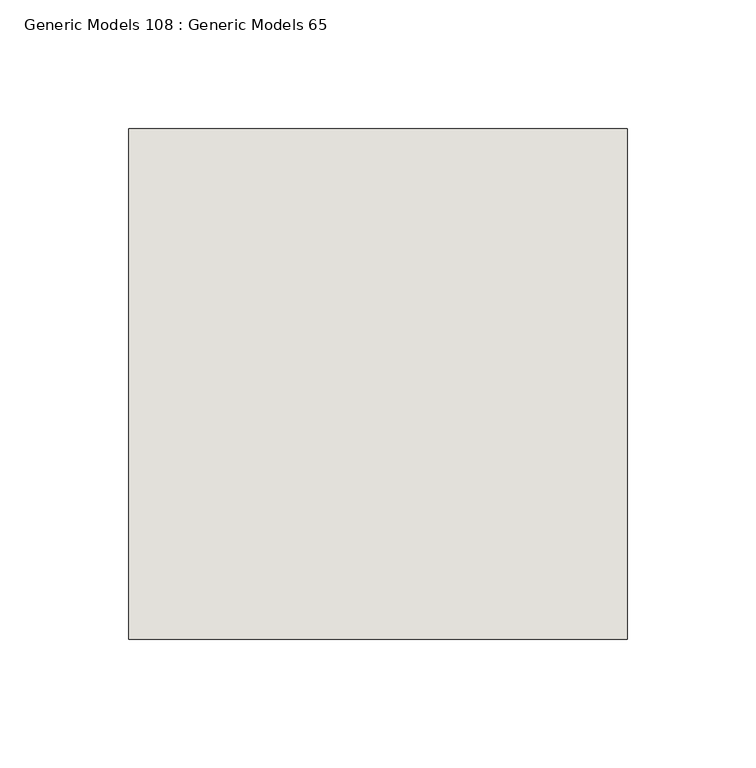
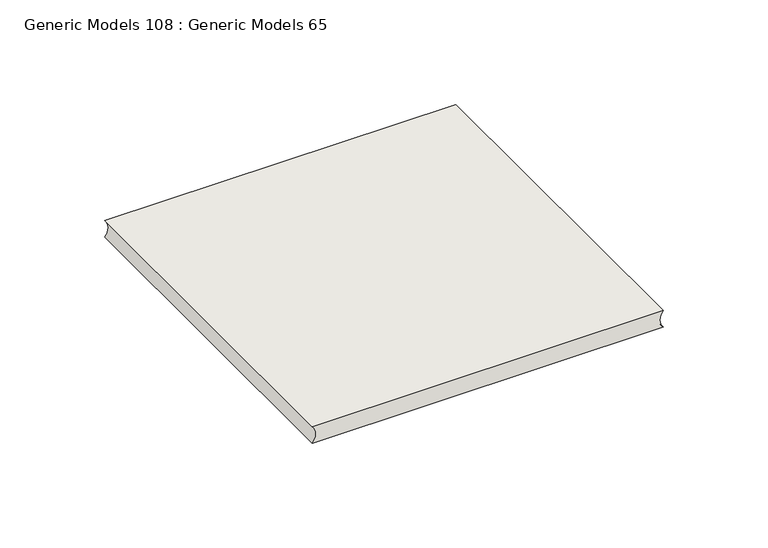
"""IFC4 building model written with IfcOpenShell, lengths in millimetres: wall geometry, Generic Models 108 : Generic Models 65."""

import ifcopenshell
import ifcopenshell.guid

model = None  # the IFC model being written
_history = None  # IfcOwnerHistory: only IFC2X3 demands one
_inside = {}  # id of a spatial element -> (the spatial element, [elements in it])
_under = {}  # id of a project, library or spatial element -> (it, [spatial elements below it])
_declared = {}  # id of a project -> (the project, [libraries it declares])
_typed = {}  # id of a type object -> (the type object, [elements of that type])
_made_of = {}  # id of a material, layer set ... -> (it, [elements and type objects made of it])


def new_model(schema):
    """Start an empty IFC model of exactly this schema.

    Asked for "IFC4X3", IfcOpenShell would pick the latest addendum, in which some entities
    have other attributes; the version numbers below select the first issue.
    IFC2X3 requires an IfcOwnerHistory on every rooted entity: one is made here for all.
    """
    global model, _history
    if schema == "IFC4X3":
        model = ifcopenshell.file(schema_version=(4, 3, 0, 0))
    else:
        model = ifcopenshell.file(schema=schema)
    _inside.clear()
    _under.clear()
    _declared.clear()
    _typed.clear()
    _made_of.clear()
    _history = None
    if model.schema == "IFC2X3":
        org = make("IfcOrganization", Name="unknown")
        user = make(
            "IfcPersonAndOrganization",
            ThePerson=make("IfcPerson", FamilyName="unknown"),
            TheOrganization=org,
        )
        app = make(
            "IfcApplication",
            ApplicationDeveloper=org,
            Version="unknown",
            ApplicationFullName="unknown",
            ApplicationIdentifier="unknown",
        )
        _history = make(
            "IfcOwnerHistory",
            OwningUser=user,
            OwningApplication=app,
            ChangeAction="ADDED",
            CreationDate=0,
        )
    return model


def make(cls, **values):
    """One entity of the class cls with the attributes given. An attribute that is None is left unset."""
    return model.create_entity(
        cls, **{name: value for name, value in values.items() if value is not None}
    )


def rooted(cls, **values):
    """An entity with a GlobalId (a new one), such as an element, a storey or a relation."""
    return make(cls, GlobalId=ifcopenshell.guid.new(), OwnerHistory=_history, **values)


def si_unit(unit_type, name, prefix=None):
    """IfcSIUnit, for example si_unit("LENGTHUNIT", "METRE", prefix="MILLI")."""
    return make("IfcSIUnit", UnitType=unit_type, Prefix=prefix, Name=name)


def assignment(units):
    """IfcUnitAssignment: the units of a project."""
    return None if units is None else make("IfcUnitAssignment", Units=units)


def point(xyz):
    """IfcCartesianPoint."""
    return None if xyz is None else make("IfcCartesianPoint", Coordinates=xyz)


def direction(xyz):
    """IfcDirection."""
    return None if xyz is None else make("IfcDirection", DirectionRatios=xyz)


def frame(location, z_axis=None, x_axis=None):
    """IfcAxis2Placement3D, a coordinate frame: its origin and axes. An axis left out is left unset."""
    return make(
        "IfcAxis2Placement3D",
        Location=point(location),
        Axis=direction(z_axis),
        RefDirection=direction(x_axis),
    )


def frame_2d(location, x_axis=None):
    """IfcAxis2Placement2D, a coordinate frame in the plane: its origin and x axis."""
    return make(
        "IfcAxis2Placement2D", Location=point(location), RefDirection=direction(x_axis)
    )


def origin():
    """The frame at (0, 0, 0) with its axes left unset."""
    return frame((0.0, 0.0, 0.0))


def place(relative_to, where):
    """IfcLocalPlacement: puts the frame where relative to a parent placement (None: the world)."""
    return make(
        "IfcLocalPlacement", PlacementRelTo=relative_to, RelativePlacement=where
    )


def context(
    kind, dimensions, precision=None, world=None, true_north=None, identifier=None
):
    """IfcGeometricRepresentationContext, for example the 3D "Model" context."""
    return make(
        "IfcGeometricRepresentationContext",
        ContextIdentifier=identifier,
        ContextType=kind,
        CoordinateSpaceDimension=dimensions,
        Precision=precision,
        WorldCoordinateSystem=world,
        TrueNorth=true_north,
    )


def project(units=None, contexts=None):
    """IfcProject with its units and contexts."""
    return rooted(
        "IfcProject",
        Name="project",
        RepresentationContexts=contexts,
        UnitsInContext=assignment(units),
    )


def spatial(cls, under=None, at=None, **own):
    """A site, building, storey or space (cls), placed at a placement, below another one or the project."""
    s = rooted(cls, ObjectPlacement=at, **own)
    if under is not None:
        _under.setdefault(under.id(), (under, []))[1].append(s)
    return s


def polyline(points):
    """IfcPolyline through the points."""
    return make("IfcPolyline", Points=[point(p) for p in points])


def circle_curve(where, radius):
    """IfcCircle in the frame where."""
    return make("IfcCircle", Position=where, Radius=radius)


def trimmed(basis, trim1, trim2, sense, master):
    """IfcTrimmedCurve: the piece of a basis curve between two trims."""
    return make(
        "IfcTrimmedCurve",
        BasisCurve=basis,
        Trim1=trim1,
        Trim2=trim2,
        SenseAgreement=sense,
        MasterRepresentation=master,
    )


def segment(curve, same_sense, transition):
    """IfcCompositeCurveSegment."""
    return make(
        "IfcCompositeCurveSegment",
        Transition=transition,
        SameSense=same_sense,
        ParentCurve=curve,
    )


def composite_curve(segments, self_intersect=None):
    """IfcCompositeCurve: segments joined end to end."""
    return make("IfcCompositeCurve", Segments=segments, SelfIntersect=self_intersect)


def outline(outer, holes=None, kind="AREA"):
    """IfcArbitraryClosedProfileDef: a profile drawn as a closed curve; with holes, ...WithVoids."""
    if holes is None:
        return make("IfcArbitraryClosedProfileDef", ProfileType=kind, OuterCurve=outer)
    return make(
        "IfcArbitraryProfileDefWithVoids",
        ProfileType=kind,
        OuterCurve=outer,
        InnerCurves=holes,
    )


def extrude(swept, where, along, depth):
    """IfcExtrudedAreaSolid: the profile swept, set in the frame where, extruded along a direction by depth."""
    return make(
        "IfcExtrudedAreaSolid",
        SweptArea=swept,
        Position=where,
        ExtrudedDirection=direction(along),
        Depth=depth,
    )


def shape(context_of_items, identifier, shape_type, items):
    """IfcShapeRepresentation: the items that make up one representation, for example the "Body"."""
    return make(
        "IfcShapeRepresentation",
        ContextOfItems=context_of_items,
        RepresentationIdentifier=identifier,
        RepresentationType=shape_type,
        Items=items,
    )


def source(mapping_origin, context_of_items, identifier, shape_type, items):
    """IfcRepresentationMap: a shape defined once, which mapped items show again and again."""
    return make(
        "IfcRepresentationMap",
        MappingOrigin=mapping_origin,
        MappedRepresentation=shape(context_of_items, identifier, shape_type, items),
    )


def transform(
    local_origin,
    x_axis=None,
    y_axis=None,
    z_axis=None,
    scale=None,
    scale2=None,
    scale3=None,
    uniform=True,
):
    """IfcCartesianTransformationOperator3D, or its non-uniform kind. x_axis, y_axis, z_axis: its Axis1, 2, 3."""
    if uniform:
        return make(
            "IfcCartesianTransformationOperator3D",
            Axis1=direction(x_axis),
            Axis2=direction(y_axis),
            LocalOrigin=point(local_origin),
            Scale=scale,
            Axis3=direction(z_axis),
        )
    return make(
        "IfcCartesianTransformationOperator3DnonUniform",
        Axis1=direction(x_axis),
        Axis2=direction(y_axis),
        LocalOrigin=point(local_origin),
        Scale=scale,
        Axis3=direction(z_axis),
        Scale2=scale2,
        Scale3=scale3,
    )


def mapped(mapping_source, mapping_target):
    """IfcMappedItem: shows the shape of a source again, moved by a transform."""
    return make(
        "IfcMappedItem", MappingSource=mapping_source, MappingTarget=mapping_target
    )


def made_of(thing, what):
    """Note that an element or type object is made of a material, layer set ...; save() writes the relation."""
    if what is not None:
        _made_of.setdefault(what.id(), (what, []))[1].append(thing)
    return thing


def element(
    cls,
    number,
    at=None,
    inside=None,
    cuts=None,
    type_object=None,
    material=None,
    context=None,
    identifier="Body",
    shape_type=None,
    held_by="IfcProductDefinitionShape",
    body=None,
    shapes=None,
    **own,
):
    """One element of the class cls, such as IfcWall. Its Tag is "e" and its number.

    at: its placement. inside: the storey or other place that contains it. cuts: it is an
    opening in that element (IfcRelVoidsElement). A single representation is given by context,
    identifier, shape_type and body (its items); several are given by shapes. held_by: the class
    of the entity that holds the representations. save() writes the other relations.
    """
    e = rooted(cls, Tag="e%d" % number, ObjectPlacement=at, **own)
    if body is not None:
        shapes = [shape(context, identifier, shape_type, body)]
    if shapes is not None:
        e.Representation = make(held_by, Representations=shapes)
    if inside is not None:
        _inside.setdefault(inside.id(), (inside, []))[1].append(e)
    if cuts is not None:
        rooted(
            "IfcRelVoidsElement", RelatingBuildingElement=cuts, RelatedOpeningElement=e
        )
    if type_object is not None:
        _typed.setdefault(type_object.id(), (type_object, []))[1].append(e)
    return made_of(e, material)


def aggregate(whole, parts):
    """IfcRelAggregates: a whole, such as a stair, and the parts it consists of."""
    return rooted("IfcRelAggregates", RelatingObject=whole, RelatedObjects=parts)


def save(model, path):
    """Write the relations noted so far, then the file.

    IfcRelAggregates (storeys below a building ...), IfcRelContainedInSpatialStructure (elements
    in a storey), IfcRelDefinesByType, IfcRelAssociatesMaterial and IfcRelDeclares: one each for
    every whole, place, type object, material and project.
    """
    for whole, parts in _under.values():
        aggregate(whole, parts)
    for where, things in _inside.values():
        rooted(
            "IfcRelContainedInSpatialStructure",
            RelatedElements=things,
            RelatingStructure=where,
        )
    for kind, things in _typed.values():
        rooted("IfcRelDefinesByType", RelatedObjects=things, RelatingType=kind)
    for what, things in _made_of.values():
        rooted("IfcRelAssociatesMaterial", RelatedObjects=things, RelatingMaterial=what)
    for by, libraries in _declared.values():
        rooted("IfcRelDeclares", RelatingContext=by, RelatedDefinitions=libraries)
    model.write(path)


def generic_models_108_generic_models_65_b715d35b(model_context):
    return source(origin(), model_context, "Body", "SweptSolid", [
        extrude(outline(composite_curve([segment(polyline([(2549.525, 375486.6125), (2549.525, 375292.9375)]), True, "CONTINUOUS"), segment(trimmed(circle_curve(frame_2d((2544.7625, 375288.0545028)), 6.8209287), [point((2549.525, 375292.9375))], [point((2540.0, 375292.9375))], True, "CARTESIAN"), True, "CONTINUOUS"), segment(polyline([(2540.0, 375292.9375), (2540.0, 375486.6125)]), True, "CONTINUOUS"), segment(trimmed(circle_curve(frame_2d((2544.7625, 375491.4954972)), 6.8209287), [point((2540.0, 375486.6125))], [point((2549.525, 375486.6125))], True, "CARTESIAN"), True, "CONTINUOUS")], self_intersect=False)), frame((0.0, 490.5375, 0.0), z_axis=(0.0, 1.0, 0.0), x_axis=(0.0, 0.0, 1.0)), (0.0, 0.0, 1.0), 198.4375),
    ])


if __name__ == "__main__":
    model = new_model("IFC4")
    model_context = context("Model", 3, world=origin())
    ifc_project = project(units=[si_unit("LENGTHUNIT", "METRE", prefix="MILLI")], contexts=[model_context])
    site = spatial("IfcSite", under=ifc_project)
    building = spatial("IfcBuilding", under=site)
    placement = place(None, origin())
    generic_models_108_generic_models_65_shape = generic_models_108_generic_models_65_b715d35b(model_context)
    element("IfcWall", 1, ObjectType="Generic Models 108 : Generic Models 65", at=placement, inside=building, context=model_context, shape_type="MappedRepresentation", body=[
        mapped(generic_models_108_generic_models_65_shape, transform((0.0, 0.0, 0.0), x_axis=(1.0, 0.0, 0.0), y_axis=(0.0, 1.0, 0.0), z_axis=(0.0, 0.0, 1.0))),
    ])
    save(model, "model.ifc")

# Revit data of these elements
# Element 1 (IfcWall, "Generic Models 108 : Generic Models 65")
#   Materials on its faces: "MORTAR JOINT"
# Materials
#   "MORTAR JOINT": class "Generic", colour RGB 120 120 120, transparency 0, Cost = 0
